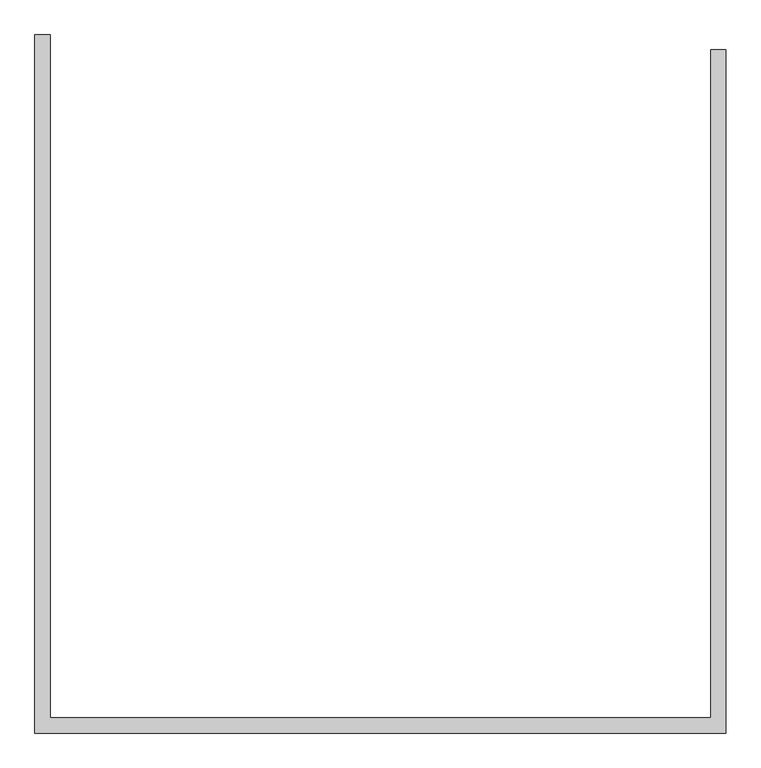
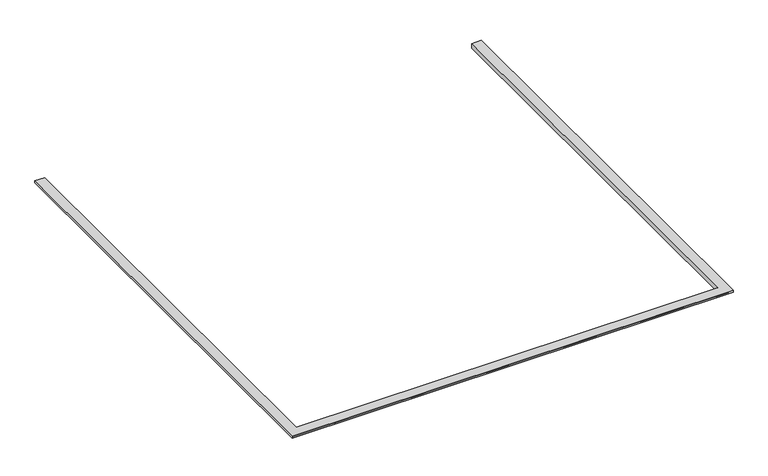
"""IFC4 building model written with IfcOpenShell, lengths in millimetres: proxy geometry, COPING MUMTY LEVEL : COPING MUMTY LEVEL."""

import ifcopenshell
import ifcopenshell.guid

model = None  # the IFC model being written
_history = None  # IfcOwnerHistory: only IFC2X3 demands one
_inside = {}  # id of a spatial element -> (the spatial element, [elements in it])
_under = {}  # id of a project, library or spatial element -> (it, [spatial elements below it])
_declared = {}  # id of a project -> (the project, [libraries it declares])
_typed = {}  # id of a type object -> (the type object, [elements of that type])
_made_of = {}  # id of a material, layer set ... -> (it, [elements and type objects made of it])


def new_model(schema):
    """Start an empty IFC model of exactly this schema.

    Asked for "IFC4X3", IfcOpenShell would pick the latest addendum, in which some entities
    have other attributes; the version numbers below select the first issue.
    IFC2X3 requires an IfcOwnerHistory on every rooted entity: one is made here for all.
    """
    global model, _history
    if schema == "IFC4X3":
        model = ifcopenshell.file(schema_version=(4, 3, 0, 0))
    else:
        model = ifcopenshell.file(schema=schema)
    _inside.clear()
    _under.clear()
    _declared.clear()
    _typed.clear()
    _made_of.clear()
    _history = None
    if model.schema == "IFC2X3":
        org = make("IfcOrganization", Name="unknown")
        user = make(
            "IfcPersonAndOrganization",
            ThePerson=make("IfcPerson", FamilyName="unknown"),
            TheOrganization=org,
        )
        app = make(
            "IfcApplication",
            ApplicationDeveloper=org,
            Version="unknown",
            ApplicationFullName="unknown",
            ApplicationIdentifier="unknown",
        )
        _history = make(
            "IfcOwnerHistory",
            OwningUser=user,
            OwningApplication=app,
            ChangeAction="ADDED",
            CreationDate=0,
        )
    return model


def make(cls, **values):
    """One entity of the class cls with the attributes given. An attribute that is None is left unset."""
    return model.create_entity(
        cls, **{name: value for name, value in values.items() if value is not None}
    )


def rooted(cls, **values):
    """An entity with a GlobalId (a new one), such as an element, a storey or a relation."""
    return make(cls, GlobalId=ifcopenshell.guid.new(), OwnerHistory=_history, **values)


def si_unit(unit_type, name, prefix=None):
    """IfcSIUnit, for example si_unit("LENGTHUNIT", "METRE", prefix="MILLI")."""
    return make("IfcSIUnit", UnitType=unit_type, Prefix=prefix, Name=name)


def assignment(units):
    """IfcUnitAssignment: the units of a project."""
    return None if units is None else make("IfcUnitAssignment", Units=units)


def point(xyz):
    """IfcCartesianPoint."""
    return None if xyz is None else make("IfcCartesianPoint", Coordinates=xyz)


def direction(xyz):
    """IfcDirection."""
    return None if xyz is None else make("IfcDirection", DirectionRatios=xyz)


def frame(location, z_axis=None, x_axis=None):
    """IfcAxis2Placement3D, a coordinate frame: its origin and axes. An axis left out is left unset."""
    return make(
        "IfcAxis2Placement3D",
        Location=point(location),
        Axis=direction(z_axis),
        RefDirection=direction(x_axis),
    )


def origin():
    """The frame at (0, 0, 0) with its axes left unset."""
    return frame((0.0, 0.0, 0.0))


def place(relative_to, where):
    """IfcLocalPlacement: puts the frame where relative to a parent placement (None: the world)."""
    return make(
        "IfcLocalPlacement", PlacementRelTo=relative_to, RelativePlacement=where
    )


def context(
    kind, dimensions, precision=None, world=None, true_north=None, identifier=None
):
    """IfcGeometricRepresentationContext, for example the 3D "Model" context."""
    return make(
        "IfcGeometricRepresentationContext",
        ContextIdentifier=identifier,
        ContextType=kind,
        CoordinateSpaceDimension=dimensions,
        Precision=precision,
        WorldCoordinateSystem=world,
        TrueNorth=true_north,
    )


def project(units=None, contexts=None):
    """IfcProject with its units and contexts."""
    return rooted(
        "IfcProject",
        Name="project",
        RepresentationContexts=contexts,
        UnitsInContext=assignment(units),
    )


def spatial(cls, under=None, at=None, **own):
    """A site, building, storey or space (cls), placed at a placement, below another one or the project."""
    s = rooted(cls, ObjectPlacement=at, **own)
    if under is not None:
        _under.setdefault(under.id(), (under, []))[1].append(s)
    return s


def polyline(points):
    """IfcPolyline through the points."""
    return make("IfcPolyline", Points=[point(p) for p in points])


def circle_curve(where, radius):
    """IfcCircle in the frame where."""
    return make("IfcCircle", Position=where, Radius=radius)


def ellipse_curve(where, semi_axis1, semi_axis2):
    """IfcEllipse in the frame where."""
    return make(
        "IfcEllipse", Position=where, SemiAxis1=semi_axis1, SemiAxis2=semi_axis2
    )


def shape(context_of_items, identifier, shape_type, items):
    """IfcShapeRepresentation: the items that make up one representation, for example the "Body"."""
    return make(
        "IfcShapeRepresentation",
        ContextOfItems=context_of_items,
        RepresentationIdentifier=identifier,
        RepresentationType=shape_type,
        Items=items,
    )


def source(mapping_origin, context_of_items, identifier, shape_type, items):
    """IfcRepresentationMap: a shape defined once, which mapped items show again and again."""
    return make(
        "IfcRepresentationMap",
        MappingOrigin=mapping_origin,
        MappedRepresentation=shape(context_of_items, identifier, shape_type, items),
    )


def transform(
    local_origin,
    x_axis=None,
    y_axis=None,
    z_axis=None,
    scale=None,
    scale2=None,
    scale3=None,
    uniform=True,
):
    """IfcCartesianTransformationOperator3D, or its non-uniform kind. x_axis, y_axis, z_axis: its Axis1, 2, 3."""
    if uniform:
        return make(
            "IfcCartesianTransformationOperator3D",
            Axis1=direction(x_axis),
            Axis2=direction(y_axis),
            LocalOrigin=point(local_origin),
            Scale=scale,
            Axis3=direction(z_axis),
        )
    return make(
        "IfcCartesianTransformationOperator3DnonUniform",
        Axis1=direction(x_axis),
        Axis2=direction(y_axis),
        LocalOrigin=point(local_origin),
        Scale=scale,
        Axis3=direction(z_axis),
        Scale2=scale2,
        Scale3=scale3,
    )


def mapped(mapping_source, mapping_target):
    """IfcMappedItem: shows the shape of a source again, moved by a transform."""
    return make(
        "IfcMappedItem", MappingSource=mapping_source, MappingTarget=mapping_target
    )


def made_of(thing, what):
    """Note that an element or type object is made of a material, layer set ...; save() writes the relation."""
    if what is not None:
        _made_of.setdefault(what.id(), (what, []))[1].append(thing)
    return thing


def element(
    cls,
    number,
    at=None,
    inside=None,
    cuts=None,
    type_object=None,
    material=None,
    context=None,
    identifier="Body",
    shape_type=None,
    held_by="IfcProductDefinitionShape",
    body=None,
    shapes=None,
    **own,
):
    """One element of the class cls, such as IfcWall. Its Tag is "e" and its number.

    at: its placement. inside: the storey or other place that contains it. cuts: it is an
    opening in that element (IfcRelVoidsElement). A single representation is given by context,
    identifier, shape_type and body (its items); several are given by shapes. held_by: the class
    of the entity that holds the representations. save() writes the other relations.
    """
    e = rooted(cls, Tag="e%d" % number, ObjectPlacement=at, **own)
    if body is not None:
        shapes = [shape(context, identifier, shape_type, body)]
    if shapes is not None:
        e.Representation = make(held_by, Representations=shapes)
    if inside is not None:
        _inside.setdefault(inside.id(), (inside, []))[1].append(e)
    if cuts is not None:
        rooted(
            "IfcRelVoidsElement", RelatingBuildingElement=cuts, RelatedOpeningElement=e
        )
    if type_object is not None:
        _typed.setdefault(type_object.id(), (type_object, []))[1].append(e)
    return made_of(e, material)


def aggregate(whole, parts):
    """IfcRelAggregates: a whole, such as a stair, and the parts it consists of."""
    return rooted("IfcRelAggregates", RelatingObject=whole, RelatedObjects=parts)


def save(model, path):
    """Write the relations noted so far, then the file.

    IfcRelAggregates (storeys below a building ...), IfcRelContainedInSpatialStructure (elements
    in a storey), IfcRelDefinesByType, IfcRelAssociatesMaterial and IfcRelDeclares: one each for
    every whole, place, type object, material and project.
    """
    for whole, parts in _under.values():
        aggregate(whole, parts)
    for where, things in _inside.values():
        rooted(
            "IfcRelContainedInSpatialStructure",
            RelatedElements=things,
            RelatingStructure=where,
        )
    for kind, things in _typed.values():
        rooted("IfcRelDefinesByType", RelatedObjects=things, RelatingType=kind)
    for what, things in _made_of.values():
        rooted("IfcRelAssociatesMaterial", RelatedObjects=things, RelatingMaterial=what)
    for by, libraries in _declared.values():
        rooted("IfcRelDeclares", RelatingContext=by, RelatedDefinitions=libraries)
    model.write(path)


def plane_surface(at):
    """IfcPlane: the flat surface through the origin of the frame at, square to its z axis."""
    return make("IfcPlane", Position=at)


def revolved_surface(curve, axis_point, axis_direction):
    """IfcSurfaceOfRevolution: the curve turned about the line through axis_point along axis_direction."""
    return make(
        "IfcSurfaceOfRevolution",
        SweptCurve=make("IfcArbitraryOpenProfileDef", ProfileType="CURVE", Curve=curve),
        AxisPosition=make("IfcAxis1Placement", Location=point(axis_point), Axis=direction(axis_direction)),
    )


def advanced_brep(points, edges, surfaces, faces):
    """IfcAdvancedBrep: a solid bounded by faces that lie on surfaces and meet in shared edges.

    An edge is (start, end): straight between two places in points (the first is 0);
    or (start, end, curve); or (start, end, curve, False) where it runs against its curve.
    A face is (place in surfaces, loops), or (place, loops, False) where it looks against
    its surface's normal. A loop lists edges by number (the first is 1), with a minus sign
    where the edge is run from its end to its start. The first loop is the outer one.
    """
    corners = [point(p) for p in points]
    vertices = [make("IfcVertexPoint", VertexGeometry=c) for c in corners]
    made = []
    for start, end, *more in edges:
        made.append(
            make(
                "IfcEdgeCurve",
                EdgeStart=vertices[start],
                EdgeEnd=vertices[end],
                EdgeGeometry=more[0] if more else make("IfcPolyline", Points=[corners[start], corners[end]]),
                SameSense=more[1] if len(more) > 1 else True,
            )
        )
    hull = []
    for where, loops, *sense in faces:
        bounds = []
        for j, loop in enumerate(loops):
            ring = [make("IfcOrientedEdge", EdgeElement=made[abs(k) - 1], Orientation=k > 0) for k in loop]
            bounds.append(
                make(
                    "IfcFaceOuterBound" if j == 0 else "IfcFaceBound",
                    Bound=make("IfcEdgeLoop", EdgeList=ring),
                    Orientation=True,
                )
            )
        hull.append(make("IfcAdvancedFace", Bounds=bounds, FaceSurface=surfaces[where], SameSense=sense[0] if sense else True))
    return make("IfcAdvancedBrep", Outer=make("IfcClosedShell", CfsFaces=hull))


def generic_models_f3d060df(model_context):
    return source(origin(), model_context, "Body", "AdvancedBrep", [
        advanced_brep(
        [(17320.1, -127.0, 9848.0), (17230.1, -127.0, 9848.0), (17230.1, -127.0, 9918.0), (17375.1, -127.0, 9918.0), (17375.1, -127.0, 9888.0), (17345.1, -127.0, 9888.0), (17345.1, -127.0, 9873.0), (17320.1, -6476.6, 9848.0), (10947.8, -6476.6, 9848.0), (10947.8, 12.7, 9848.0), (11037.8, 12.7, 9848.0), (11037.8, -6386.6, 9848.0), (17230.1, -6386.6, 9848.0), (17230.1, -6386.6, 9918.0), (11037.8, -6386.6, 9918.0), (11037.8, 12.7, 9918.0), (10892.8, 12.7, 9918.0), (10892.8, -6531.6, 9918.0), (17375.1, -6531.6, 9918.0), (17375.1, -6531.6, 9888.0), (10892.8, -6531.6, 9888.0), (10892.8, 12.7, 9888.0), (10922.8, 12.7, 9888.0), (10922.8, -6501.6, 9888.0), (17345.1, -6501.6, 9888.0), (17345.1, -6501.6, 9873.0), (10922.8, -6501.6, 9873.0), (10922.8, 12.7, 9873.0)],
        [
            (0, 1),
            (1, 2),
            (2, 3),
            (3, 4),
            (4, 5),
            (5, 6),
            (6, 0, circle_curve(frame((17345.1, -127.0, 9848.0), z_axis=(0.0, -1.0, 0.0), x_axis=(1.0, 0.0, 0.0)), 25.0)),
            (0, 7),
            (7, 8),
            (8, 9),
            (9, 10),
            (10, 11),
            (11, 12),
            (12, 1),
            (12, 13),
            (13, 2),
            (13, 14),
            (14, 15),
            (15, 16),
            (16, 17),
            (17, 18),
            (18, 3),
            (18, 19),
            (19, 4),
            (19, 20),
            (20, 21),
            (21, 22),
            (22, 23),
            (23, 24),
            (24, 5),
            (24, 25),
            (25, 6),
            (25, 7, ellipse_curve(frame((17345.1, -6501.6, 9848.0), z_axis=(-0.7071067811865475, -0.7071067811865475, 0.0), x_axis=(0.7071067811865474, -0.7071067811865476, 0.0)), 35.3553391, 25.0)),
            (11, 14),
            (17, 20),
            (23, 26),
            (26, 25),
            (26, 8, ellipse_curve(frame((10922.8, -6501.6, 9848.0), z_axis=(-0.7071067811865475, 0.7071067811865475, 0.0), x_axis=(-0.7071067811865476, -0.7071067811865474, 0.0)), 35.3553391, 25.0)),
            (9, 27, circle_curve(frame((10922.8, 12.7, 9848.0), z_axis=(0.0, -1.0, 0.0), x_axis=(-1.0, 0.0, 0.0)), 25.0)),
            (27, 22),
            (21, 16),
            (15, 10),
            (27, 26),
        ],
        [
            plane_surface(frame((17310.1, -127.0, 9848.0), z_axis=(0.0, 1.0, 0.0), x_axis=(0.0, 0.0, 1.0))),
            plane_surface(frame((17310.1, -127.0, 9848.0), z_axis=(0.0, 0.0, -1.0), x_axis=(0.0, -1.0, 0.0))),
            plane_surface(frame((17230.1, -127.0, 9848.0), z_axis=(-1.0, 0.0, 0.0), x_axis=(0.0, -1.0, 0.0))),
            plane_surface(frame((17230.1, -127.0, 9918.0), z_axis=(0.0, 0.0, 1.0), x_axis=(0.0, -1.0, 0.0))),
            plane_surface(frame((17375.1, -127.0, 9918.0), z_axis=(1.0, 0.0, 0.0), x_axis=(0.0, -1.0, 0.0))),
            plane_surface(frame((17375.1, -127.0, 9888.0), z_axis=(0.0, 0.0, -1.0), x_axis=(0.0, -1.0, 0.0))),
            plane_surface(frame((17345.1, -127.0, 9888.0), z_axis=(1.0, 0.0, 0.0), x_axis=(0.0, -1.0, 0.0))),
            revolved_surface(polyline([(17370.1, -6526.60000002876, 9848.0), (17370.1, -127.0, 9848.0)]), (17345.1, -127.0, 9848.0), (0.0, -1.0, 0.0)),
            plane_surface(frame((17230.1, -6386.6, 9848.0), z_axis=(0.0, 1.0, 0.0), x_axis=(-1.0, 0.0, 0.0))),
            plane_surface(frame((17375.1, -6531.6, 9918.0), z_axis=(0.0, -1.0, 0.0), x_axis=(-1.0, 0.0, 0.0))),
            plane_surface(frame((17345.1, -6501.6, 9888.0), z_axis=(0.0, -1.0, 0.0), x_axis=(-1.0, 0.0, 0.0))),
            revolved_surface(polyline([(10897.79999997124, -6526.6, 9848.0), (17370.100000028757, -6526.6, 9848.0)]), (17310.1, -6501.6, 9848.0), (-1.0, 0.0, 0.0)),
            plane_surface(frame((10957.8, 12.7, 9848.0), z_axis=(0.0, 1.0, 0.0), x_axis=(0.0, 0.0, 1.0))),
            plane_surface(frame((11037.8, -6386.6, 9848.0), z_axis=(1.0, 0.0, 0.0), x_axis=(0.0, 1.0, 0.0))),
            plane_surface(frame((10892.8, -6531.6, 9918.0), z_axis=(-1.0, 0.0, 0.0), x_axis=(0.0, 1.0, 0.0))),
            plane_surface(frame((10922.8, -6501.6, 9888.0), z_axis=(-1.0, 0.0, 0.0), x_axis=(0.0, 1.0, 0.0))),
            revolved_surface(polyline([(10897.8, 12.699999999999818, 9848.0), (10897.8, -6526.60000002876, 9848.0)]), (10922.8, -6466.6, 9848.0), (0.0, 1.0, 0.0)),
        ],
        [
            (0, [[1, 2, 3, 4, 5, 6, 7]]),
            (1, [[8, 9, 10, 11, 12, 13, 14, -1]]),
            (2, [[-2, -14, 15, 16]]),
            (3, [[-3, -16, 17, 18, 19, 20, 21, 22]]),
            (4, [[-4, -22, 23, 24]]),
            (5, [[-5, -24, 25, 26, 27, 28, 29, 30]]),
            (6, [[-6, -30, 31, 32]]),
            (7, [[-7, -32, 33, -8]]),
            (8, [[-15, -13, 34, -17]]),
            (9, [[-23, -21, 35, -25]]),
            (10, [[-31, -29, 36, 37]]),
            (11, [[-33, -37, 38, -9]]),
            (12, [[-11, 39, 40, -27, 41, -19, 42]]),
            (13, [[-34, -12, -42, -18]]),
            (14, [[-35, -20, -41, -26]]),
            (15, [[-36, -28, -40, 43]]),
            (16, [[-38, -43, -39, -10]]),
        ],
    ),
    ])


if __name__ == "__main__":
    model = new_model("IFC4")
    model_context = context("Model", 3, world=origin())
    ifc_project = project(units=[si_unit("LENGTHUNIT", "METRE", prefix="MILLI")], contexts=[model_context])
    site = spatial("IfcSite", under=ifc_project)
    building = spatial("IfcBuilding", under=site)
    placement = place(None, origin())
    generic_models_shape = generic_models_f3d060df(model_context)
    element("IfcBuildingElementProxy", 1, Name="COPING MUMTY LEVEL : COPING MUMTY LEVEL", ObjectType="COPING MUMTY LEVEL : COPING MUMTY LEVEL", at=placement, inside=building, context=model_context, shape_type="MappedRepresentation", body=[
        mapped(generic_models_shape, transform((0.0, 0.0, 0.0), x_axis=(1.0, 0.0, 0.0), y_axis=(0.0, 1.0, 0.0), z_axis=(0.0, 0.0, 1.0))),
    ])
    save(model, "model.ifc")

# Revit data of these elements
# Element 1 (IfcBuildingElementProxy, "COPING MUMTY LEVEL : COPING MUMTY LEVEL")
#   Materials on its faces: "wooden-3"
# Materials
#   "wooden-3": class "Generic", colour RGB 120 120 120, transparency 0, Cost = 0
